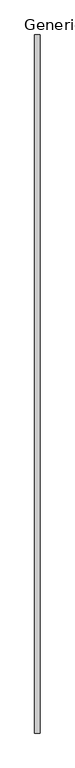
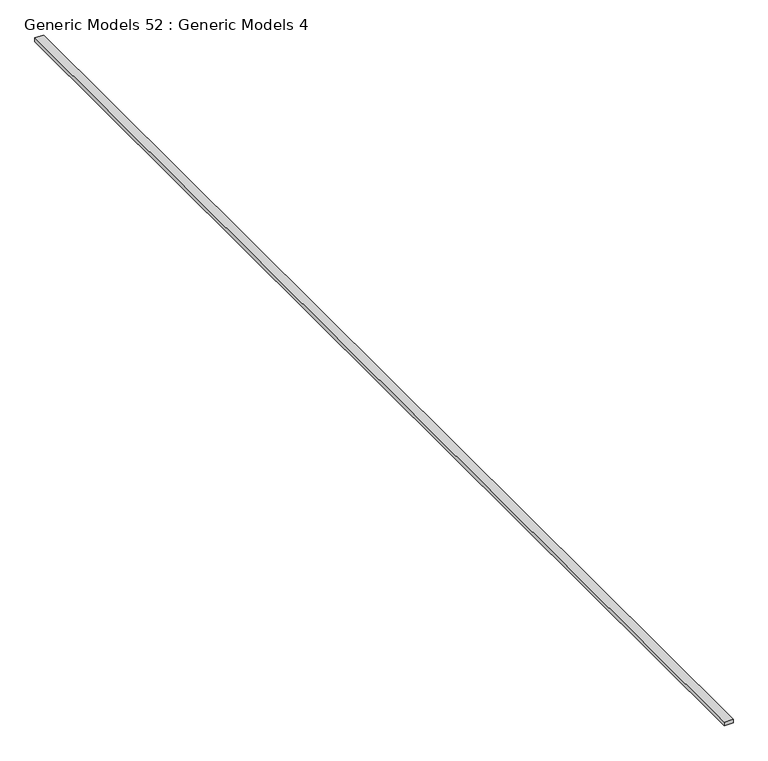
"""IFC4 building model written with IfcOpenShell, lengths in millimetres: proxy geometry, Generic Models 52 : Generic Models 4."""

import ifcopenshell
import ifcopenshell.guid

model = None  # the IFC model being written
_history = None  # IfcOwnerHistory: only IFC2X3 demands one
_inside = {}  # id of a spatial element -> (the spatial element, [elements in it])
_under = {}  # id of a project, library or spatial element -> (it, [spatial elements below it])
_declared = {}  # id of a project -> (the project, [libraries it declares])
_typed = {}  # id of a type object -> (the type object, [elements of that type])
_made_of = {}  # id of a material, layer set ... -> (it, [elements and type objects made of it])


def new_model(schema):
    """Start an empty IFC model of exactly this schema.

    Asked for "IFC4X3", IfcOpenShell would pick the latest addendum, in which some entities
    have other attributes; the version numbers below select the first issue.
    IFC2X3 requires an IfcOwnerHistory on every rooted entity: one is made here for all.
    """
    global model, _history
    if schema == "IFC4X3":
        model = ifcopenshell.file(schema_version=(4, 3, 0, 0))
    else:
        model = ifcopenshell.file(schema=schema)
    _inside.clear()
    _under.clear()
    _declared.clear()
    _typed.clear()
    _made_of.clear()
    _history = None
    if model.schema == "IFC2X3":
        org = make("IfcOrganization", Name="unknown")
        user = make(
            "IfcPersonAndOrganization",
            ThePerson=make("IfcPerson", FamilyName="unknown"),
            TheOrganization=org,
        )
        app = make(
            "IfcApplication",
            ApplicationDeveloper=org,
            Version="unknown",
            ApplicationFullName="unknown",
            ApplicationIdentifier="unknown",
        )
        _history = make(
            "IfcOwnerHistory",
            OwningUser=user,
            OwningApplication=app,
            ChangeAction="ADDED",
            CreationDate=0,
        )
    return model


def make(cls, **values):
    """One entity of the class cls with the attributes given. An attribute that is None is left unset."""
    return model.create_entity(
        cls, **{name: value for name, value in values.items() if value is not None}
    )


def rooted(cls, **values):
    """An entity with a GlobalId (a new one), such as an element, a storey or a relation."""
    return make(cls, GlobalId=ifcopenshell.guid.new(), OwnerHistory=_history, **values)


def si_unit(unit_type, name, prefix=None):
    """IfcSIUnit, for example si_unit("LENGTHUNIT", "METRE", prefix="MILLI")."""
    return make("IfcSIUnit", UnitType=unit_type, Prefix=prefix, Name=name)


def assignment(units):
    """IfcUnitAssignment: the units of a project."""
    return None if units is None else make("IfcUnitAssignment", Units=units)


def point(xyz):
    """IfcCartesianPoint."""
    return None if xyz is None else make("IfcCartesianPoint", Coordinates=xyz)


def direction(xyz):
    """IfcDirection."""
    return None if xyz is None else make("IfcDirection", DirectionRatios=xyz)


def frame(location, z_axis=None, x_axis=None):
    """IfcAxis2Placement3D, a coordinate frame: its origin and axes. An axis left out is left unset."""
    return make(
        "IfcAxis2Placement3D",
        Location=point(location),
        Axis=direction(z_axis),
        RefDirection=direction(x_axis),
    )


def origin():
    """The frame at (0, 0, 0) with its axes left unset."""
    return frame((0.0, 0.0, 0.0))


def place(relative_to, where):
    """IfcLocalPlacement: puts the frame where relative to a parent placement (None: the world)."""
    return make(
        "IfcLocalPlacement", PlacementRelTo=relative_to, RelativePlacement=where
    )


def context(
    kind, dimensions, precision=None, world=None, true_north=None, identifier=None
):
    """IfcGeometricRepresentationContext, for example the 3D "Model" context."""
    return make(
        "IfcGeometricRepresentationContext",
        ContextIdentifier=identifier,
        ContextType=kind,
        CoordinateSpaceDimension=dimensions,
        Precision=precision,
        WorldCoordinateSystem=world,
        TrueNorth=true_north,
    )


def project(units=None, contexts=None):
    """IfcProject with its units and contexts."""
    return rooted(
        "IfcProject",
        Name="project",
        RepresentationContexts=contexts,
        UnitsInContext=assignment(units),
    )


def spatial(cls, under=None, at=None, **own):
    """A site, building, storey or space (cls), placed at a placement, below another one or the project."""
    s = rooted(cls, ObjectPlacement=at, **own)
    if under is not None:
        _under.setdefault(under.id(), (under, []))[1].append(s)
    return s


def polyline(points):
    """IfcPolyline through the points."""
    return make("IfcPolyline", Points=[point(p) for p in points])


def outline(outer, holes=None, kind="AREA"):
    """IfcArbitraryClosedProfileDef: a profile drawn as a closed curve; with holes, ...WithVoids."""
    if holes is None:
        return make("IfcArbitraryClosedProfileDef", ProfileType=kind, OuterCurve=outer)
    return make(
        "IfcArbitraryProfileDefWithVoids",
        ProfileType=kind,
        OuterCurve=outer,
        InnerCurves=holes,
    )


def extrude(swept, where, along, depth):
    """IfcExtrudedAreaSolid: the profile swept, set in the frame where, extruded along a direction by depth."""
    return make(
        "IfcExtrudedAreaSolid",
        SweptArea=swept,
        Position=where,
        ExtrudedDirection=direction(along),
        Depth=depth,
    )


def shape(context_of_items, identifier, shape_type, items):
    """IfcShapeRepresentation: the items that make up one representation, for example the "Body"."""
    return make(
        "IfcShapeRepresentation",
        ContextOfItems=context_of_items,
        RepresentationIdentifier=identifier,
        RepresentationType=shape_type,
        Items=items,
    )


def source(mapping_origin, context_of_items, identifier, shape_type, items):
    """IfcRepresentationMap: a shape defined once, which mapped items show again and again."""
    return make(
        "IfcRepresentationMap",
        MappingOrigin=mapping_origin,
        MappedRepresentation=shape(context_of_items, identifier, shape_type, items),
    )


def transform(
    local_origin,
    x_axis=None,
    y_axis=None,
    z_axis=None,
    scale=None,
    scale2=None,
    scale3=None,
    uniform=True,
):
    """IfcCartesianTransformationOperator3D, or its non-uniform kind. x_axis, y_axis, z_axis: its Axis1, 2, 3."""
    if uniform:
        return make(
            "IfcCartesianTransformationOperator3D",
            Axis1=direction(x_axis),
            Axis2=direction(y_axis),
            LocalOrigin=point(local_origin),
            Scale=scale,
            Axis3=direction(z_axis),
        )
    return make(
        "IfcCartesianTransformationOperator3DnonUniform",
        Axis1=direction(x_axis),
        Axis2=direction(y_axis),
        LocalOrigin=point(local_origin),
        Scale=scale,
        Axis3=direction(z_axis),
        Scale2=scale2,
        Scale3=scale3,
    )


def mapped(mapping_source, mapping_target):
    """IfcMappedItem: shows the shape of a source again, moved by a transform."""
    return make(
        "IfcMappedItem", MappingSource=mapping_source, MappingTarget=mapping_target
    )


def made_of(thing, what):
    """Note that an element or type object is made of a material, layer set ...; save() writes the relation."""
    if what is not None:
        _made_of.setdefault(what.id(), (what, []))[1].append(thing)
    return thing


def element(
    cls,
    number,
    at=None,
    inside=None,
    cuts=None,
    type_object=None,
    material=None,
    context=None,
    identifier="Body",
    shape_type=None,
    held_by="IfcProductDefinitionShape",
    body=None,
    shapes=None,
    **own,
):
    """One element of the class cls, such as IfcWall. Its Tag is "e" and its number.

    at: its placement. inside: the storey or other place that contains it. cuts: it is an
    opening in that element (IfcRelVoidsElement). A single representation is given by context,
    identifier, shape_type and body (its items); several are given by shapes. held_by: the class
    of the entity that holds the representations. save() writes the other relations.
    """
    e = rooted(cls, Tag="e%d" % number, ObjectPlacement=at, **own)
    if body is not None:
        shapes = [shape(context, identifier, shape_type, body)]
    if shapes is not None:
        e.Representation = make(held_by, Representations=shapes)
    if inside is not None:
        _inside.setdefault(inside.id(), (inside, []))[1].append(e)
    if cuts is not None:
        rooted(
            "IfcRelVoidsElement", RelatingBuildingElement=cuts, RelatedOpeningElement=e
        )
    if type_object is not None:
        _typed.setdefault(type_object.id(), (type_object, []))[1].append(e)
    return made_of(e, material)


def aggregate(whole, parts):
    """IfcRelAggregates: a whole, such as a stair, and the parts it consists of."""
    return rooted("IfcRelAggregates", RelatingObject=whole, RelatedObjects=parts)


def save(model, path):
    """Write the relations noted so far, then the file.

    IfcRelAggregates (storeys below a building ...), IfcRelContainedInSpatialStructure (elements
    in a storey), IfcRelDefinesByType, IfcRelAssociatesMaterial and IfcRelDeclares: one each for
    every whole, place, type object, material and project.
    """
    for whole, parts in _under.values():
        aggregate(whole, parts)
    for where, things in _inside.values():
        rooted(
            "IfcRelContainedInSpatialStructure",
            RelatedElements=things,
            RelatingStructure=where,
        )
    for kind, things in _typed.values():
        rooted("IfcRelDefinesByType", RelatedObjects=things, RelatingType=kind)
    for what, things in _made_of.values():
        rooted("IfcRelAssociatesMaterial", RelatedObjects=things, RelatingMaterial=what)
    for by, libraries in _declared.values():
        rooted("IfcRelDeclares", RelatingContext=by, RelatedDefinitions=libraries)
    model.write(path)


def generic_models_52_generic_models_4_03f68ce8(model_context):
    return source(origin(), model_context, "Body", "SweptSolid", [
        extrude(outline(polyline([(127040.4410334, 7095.9513704), (127040.4410334, 7235.6513704), (127097.68533, 7235.6513704), (127103.5061634, 7095.9513704), (127040.4410334, 7095.9513704)])), frame((0.0, -6864.9230338, 0.0), z_axis=(0.0, 1.0, 0.0), x_axis=(0.0, 0.0, 1.0)), (0.0, 0.0, 1.0), 18643.6),
    ])


if __name__ == "__main__":
    model = new_model("IFC4")
    model_context = context("Model", 3, world=origin())
    ifc_project = project(units=[si_unit("LENGTHUNIT", "METRE", prefix="MILLI")], contexts=[model_context])
    site = spatial("IfcSite", under=ifc_project)
    building = spatial("IfcBuilding", under=site)
    placement = place(None, origin())
    generic_models_52_generic_models_4_shape = generic_models_52_generic_models_4_03f68ce8(model_context)
    element("IfcBuildingElementProxy", 1, Name="Generic Models 52 : Generic Models 4", ObjectType="Generic Models 52 : Generic Models 4", at=placement, inside=building, context=model_context, shape_type="MappedRepresentation", body=[
        mapped(generic_models_52_generic_models_4_shape, transform((0.0, 0.0, 0.0), x_axis=(1.0, 0.0, 0.0), y_axis=(0.0, 1.0, 0.0), z_axis=(0.0, 0.0, 1.0))),
    ])
    save(model, "model.ifc")

# Revit data of these elements
# Element 1 (IfcBuildingElementProxy, "Generic Models 52 : Generic Models 4")
#   Materials on its faces: "_2X BLOCKING AS REQUIRED"
# Materials
#   "_2X BLOCKING AS REQUIRED": class "Generic", colour RGB 177 130 114, transparency 0, Cost = 0
